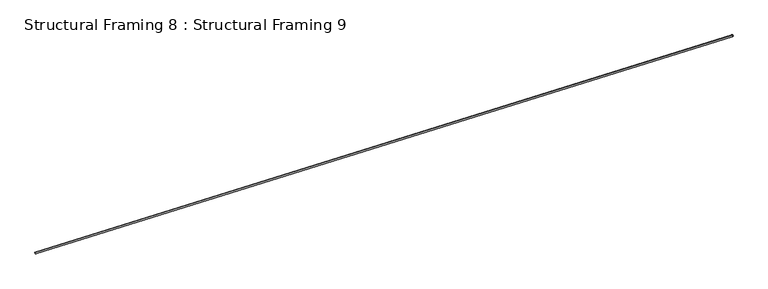
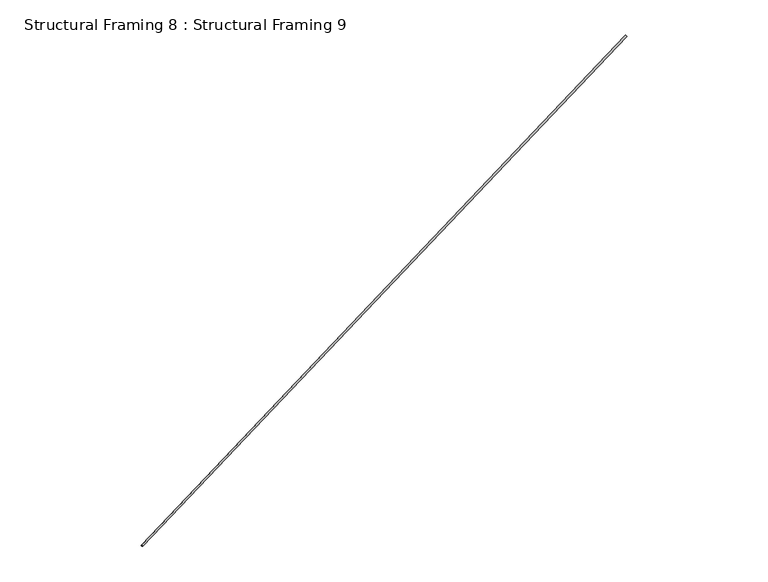
"""IFC4 building model written with IfcOpenShell, lengths in millimetres: beam geometry, Structural Framing 8 : Structural Framing 9."""

import ifcopenshell
import ifcopenshell.guid

model = None  # the IFC model being written
_history = None  # IfcOwnerHistory: only IFC2X3 demands one
_inside = {}  # id of a spatial element -> (the spatial element, [elements in it])
_under = {}  # id of a project, library or spatial element -> (it, [spatial elements below it])
_declared = {}  # id of a project -> (the project, [libraries it declares])
_typed = {}  # id of a type object -> (the type object, [elements of that type])
_made_of = {}  # id of a material, layer set ... -> (it, [elements and type objects made of it])


def new_model(schema):
    """Start an empty IFC model of exactly this schema.

    Asked for "IFC4X3", IfcOpenShell would pick the latest addendum, in which some entities
    have other attributes; the version numbers below select the first issue.
    IFC2X3 requires an IfcOwnerHistory on every rooted entity: one is made here for all.
    """
    global model, _history
    if schema == "IFC4X3":
        model = ifcopenshell.file(schema_version=(4, 3, 0, 0))
    else:
        model = ifcopenshell.file(schema=schema)
    _inside.clear()
    _under.clear()
    _declared.clear()
    _typed.clear()
    _made_of.clear()
    _history = None
    if model.schema == "IFC2X3":
        org = make("IfcOrganization", Name="unknown")
        user = make(
            "IfcPersonAndOrganization",
            ThePerson=make("IfcPerson", FamilyName="unknown"),
            TheOrganization=org,
        )
        app = make(
            "IfcApplication",
            ApplicationDeveloper=org,
            Version="unknown",
            ApplicationFullName="unknown",
            ApplicationIdentifier="unknown",
        )
        _history = make(
            "IfcOwnerHistory",
            OwningUser=user,
            OwningApplication=app,
            ChangeAction="ADDED",
            CreationDate=0,
        )
    return model


def make(cls, **values):
    """One entity of the class cls with the attributes given. An attribute that is None is left unset."""
    return model.create_entity(
        cls, **{name: value for name, value in values.items() if value is not None}
    )


def rooted(cls, **values):
    """An entity with a GlobalId (a new one), such as an element, a storey or a relation."""
    return make(cls, GlobalId=ifcopenshell.guid.new(), OwnerHistory=_history, **values)


def si_unit(unit_type, name, prefix=None):
    """IfcSIUnit, for example si_unit("LENGTHUNIT", "METRE", prefix="MILLI")."""
    return make("IfcSIUnit", UnitType=unit_type, Prefix=prefix, Name=name)


def assignment(units):
    """IfcUnitAssignment: the units of a project."""
    return None if units is None else make("IfcUnitAssignment", Units=units)


def point(xyz):
    """IfcCartesianPoint."""
    return None if xyz is None else make("IfcCartesianPoint", Coordinates=xyz)


def direction(xyz):
    """IfcDirection."""
    return None if xyz is None else make("IfcDirection", DirectionRatios=xyz)


def frame(location, z_axis=None, x_axis=None):
    """IfcAxis2Placement3D, a coordinate frame: its origin and axes. An axis left out is left unset."""
    return make(
        "IfcAxis2Placement3D",
        Location=point(location),
        Axis=direction(z_axis),
        RefDirection=direction(x_axis),
    )


def frame_2d(location, x_axis=None):
    """IfcAxis2Placement2D, a coordinate frame in the plane: its origin and x axis."""
    return make(
        "IfcAxis2Placement2D", Location=point(location), RefDirection=direction(x_axis)
    )


def origin():
    """The frame at (0, 0, 0) with its axes left unset."""
    return frame((0.0, 0.0, 0.0))


def origin_2d():
    """The frame at (0, 0) in the plane with its x axis left unset."""
    return frame_2d((0.0, 0.0))


def place(relative_to, where):
    """IfcLocalPlacement: puts the frame where relative to a parent placement (None: the world)."""
    return make(
        "IfcLocalPlacement", PlacementRelTo=relative_to, RelativePlacement=where
    )


def context(
    kind, dimensions, precision=None, world=None, true_north=None, identifier=None
):
    """IfcGeometricRepresentationContext, for example the 3D "Model" context."""
    return make(
        "IfcGeometricRepresentationContext",
        ContextIdentifier=identifier,
        ContextType=kind,
        CoordinateSpaceDimension=dimensions,
        Precision=precision,
        WorldCoordinateSystem=world,
        TrueNorth=true_north,
    )


def project(units=None, contexts=None):
    """IfcProject with its units and contexts."""
    return rooted(
        "IfcProject",
        Name="project",
        RepresentationContexts=contexts,
        UnitsInContext=assignment(units),
    )


def spatial(cls, under=None, at=None, **own):
    """A site, building, storey or space (cls), placed at a placement, below another one or the project."""
    s = rooted(cls, ObjectPlacement=at, **own)
    if under is not None:
        _under.setdefault(under.id(), (under, []))[1].append(s)
    return s


def circle_curve(where, radius):
    """IfcCircle in the frame where."""
    return make("IfcCircle", Position=where, Radius=radius)


def trimmed(basis, trim1, trim2, sense, master):
    """IfcTrimmedCurve: the piece of a basis curve between two trims."""
    return make(
        "IfcTrimmedCurve",
        BasisCurve=basis,
        Trim1=trim1,
        Trim2=trim2,
        SenseAgreement=sense,
        MasterRepresentation=master,
    )


def segment(curve, same_sense, transition):
    """IfcCompositeCurveSegment."""
    return make(
        "IfcCompositeCurveSegment",
        Transition=transition,
        SameSense=same_sense,
        ParentCurve=curve,
    )


def composite_curve(segments, self_intersect=None):
    """IfcCompositeCurve: segments joined end to end."""
    return make("IfcCompositeCurve", Segments=segments, SelfIntersect=self_intersect)


def outline(outer, holes=None, kind="AREA"):
    """IfcArbitraryClosedProfileDef: a profile drawn as a closed curve; with holes, ...WithVoids."""
    if holes is None:
        return make("IfcArbitraryClosedProfileDef", ProfileType=kind, OuterCurve=outer)
    return make(
        "IfcArbitraryProfileDefWithVoids",
        ProfileType=kind,
        OuterCurve=outer,
        InnerCurves=holes,
    )


def extrude(swept, where, along, depth):
    """IfcExtrudedAreaSolid: the profile swept, set in the frame where, extruded along a direction by depth."""
    return make(
        "IfcExtrudedAreaSolid",
        SweptArea=swept,
        Position=where,
        ExtrudedDirection=direction(along),
        Depth=depth,
    )


def shape(context_of_items, identifier, shape_type, items):
    """IfcShapeRepresentation: the items that make up one representation, for example the "Body"."""
    return make(
        "IfcShapeRepresentation",
        ContextOfItems=context_of_items,
        RepresentationIdentifier=identifier,
        RepresentationType=shape_type,
        Items=items,
    )


def source(mapping_origin, context_of_items, identifier, shape_type, items):
    """IfcRepresentationMap: a shape defined once, which mapped items show again and again."""
    return make(
        "IfcRepresentationMap",
        MappingOrigin=mapping_origin,
        MappedRepresentation=shape(context_of_items, identifier, shape_type, items),
    )


def transform(
    local_origin,
    x_axis=None,
    y_axis=None,
    z_axis=None,
    scale=None,
    scale2=None,
    scale3=None,
    uniform=True,
):
    """IfcCartesianTransformationOperator3D, or its non-uniform kind. x_axis, y_axis, z_axis: its Axis1, 2, 3."""
    if uniform:
        return make(
            "IfcCartesianTransformationOperator3D",
            Axis1=direction(x_axis),
            Axis2=direction(y_axis),
            LocalOrigin=point(local_origin),
            Scale=scale,
            Axis3=direction(z_axis),
        )
    return make(
        "IfcCartesianTransformationOperator3DnonUniform",
        Axis1=direction(x_axis),
        Axis2=direction(y_axis),
        LocalOrigin=point(local_origin),
        Scale=scale,
        Axis3=direction(z_axis),
        Scale2=scale2,
        Scale3=scale3,
    )


def mapped(mapping_source, mapping_target):
    """IfcMappedItem: shows the shape of a source again, moved by a transform."""
    return make(
        "IfcMappedItem", MappingSource=mapping_source, MappingTarget=mapping_target
    )


def made_of(thing, what):
    """Note that an element or type object is made of a material, layer set ...; save() writes the relation."""
    if what is not None:
        _made_of.setdefault(what.id(), (what, []))[1].append(thing)
    return thing


def element(
    cls,
    number,
    at=None,
    inside=None,
    cuts=None,
    type_object=None,
    material=None,
    context=None,
    identifier="Body",
    shape_type=None,
    held_by="IfcProductDefinitionShape",
    body=None,
    shapes=None,
    **own,
):
    """One element of the class cls, such as IfcWall. Its Tag is "e" and its number.

    at: its placement. inside: the storey or other place that contains it. cuts: it is an
    opening in that element (IfcRelVoidsElement). A single representation is given by context,
    identifier, shape_type and body (its items); several are given by shapes. held_by: the class
    of the entity that holds the representations. save() writes the other relations.
    """
    e = rooted(cls, Tag="e%d" % number, ObjectPlacement=at, **own)
    if body is not None:
        shapes = [shape(context, identifier, shape_type, body)]
    if shapes is not None:
        e.Representation = make(held_by, Representations=shapes)
    if inside is not None:
        _inside.setdefault(inside.id(), (inside, []))[1].append(e)
    if cuts is not None:
        rooted(
            "IfcRelVoidsElement", RelatingBuildingElement=cuts, RelatedOpeningElement=e
        )
    if type_object is not None:
        _typed.setdefault(type_object.id(), (type_object, []))[1].append(e)
    return made_of(e, material)


def aggregate(whole, parts):
    """IfcRelAggregates: a whole, such as a stair, and the parts it consists of."""
    return rooted("IfcRelAggregates", RelatingObject=whole, RelatedObjects=parts)


def save(model, path):
    """Write the relations noted so far, then the file.

    IfcRelAggregates (storeys below a building ...), IfcRelContainedInSpatialStructure (elements
    in a storey), IfcRelDefinesByType, IfcRelAssociatesMaterial and IfcRelDeclares: one each for
    every whole, place, type object, material and project.
    """
    for whole, parts in _under.values():
        aggregate(whole, parts)
    for where, things in _inside.values():
        rooted(
            "IfcRelContainedInSpatialStructure",
            RelatedElements=things,
            RelatingStructure=where,
        )
    for kind, things in _typed.values():
        rooted("IfcRelDefinesByType", RelatedObjects=things, RelatingType=kind)
    for what, things in _made_of.values():
        rooted("IfcRelAssociatesMaterial", RelatedObjects=things, RelatingMaterial=what)
    for by, libraries in _declared.values():
        rooted("IfcRelDeclares", RelatingContext=by, RelatedDefinitions=libraries)
    model.write(path)


def structural_framing_8_structural_framing_9_a7c71935(model_context):
    return source(origin(), model_context, "Body", "SweptSolid", [
        extrude(outline(composite_curve([segment(trimmed(circle_curve(origin_2d(), 6.35), [point((0.0, -6.35))], [point((0.0, 6.35))], False, "CARTESIAN"), True, "CONTINUOUS"), segment(trimmed(circle_curve(origin_2d(), 6.35), [point((0.0, 6.35))], [point((0.0, -6.35))], False, "CARTESIAN"), True, "CONTINUOUS")], self_intersect=False)), frame((12608.4580052, 2538.5077975, 2956.2008394), z_axis=(0.8989286779363534, 0.28046158673269594, 0.3365539040792405), x_axis=(0.0, 0.7682212795973775, -0.6401843996644779)), (0.0, 0.0, 1.0), 5845.7129347),
    ])


if __name__ == "__main__":
    model = new_model("IFC4")
    model_context = context("Model", 3, world=origin())
    ifc_project = project(units=[si_unit("LENGTHUNIT", "METRE", prefix="MILLI")], contexts=[model_context])
    site = spatial("IfcSite", under=ifc_project)
    building = spatial("IfcBuilding", under=site)
    placement = place(None, origin())
    structural_framing_8_structural_framing_9_shape = structural_framing_8_structural_framing_9_a7c71935(model_context)
    element("IfcBeam", 1, ObjectType="Structural Framing 8 : Structural Framing 9", at=placement, inside=building, context=model_context, shape_type="MappedRepresentation", body=[
        mapped(structural_framing_8_structural_framing_9_shape, transform((0.0, 0.0, 0.0), x_axis=(1.0, 0.0, 0.0), y_axis=(0.0, 1.0, 0.0), z_axis=(0.0, 0.0, 1.0))),
    ])
    save(model, "model.ifc")

# Revit data of these elements
# Type "Structural Framing 8 : Structural Framing 9"
#   Structural Material [instance default] = EXISTING LATERAL BRACING (1/4" CABLE)
# Element 1 (IfcBeam, "Structural Framing 8 : Structural Framing 9")
#   Materials on its faces: "EXISTING LATERAL BRACING (1/4\" CABLE)"
# Materials
#   "EXISTING LATERAL BRACING (1/4\" CABLE)": class "Generic", colour RGB 120 120 120, transparency 0, Cost = 0
